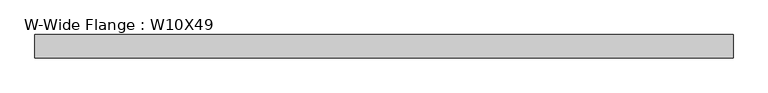
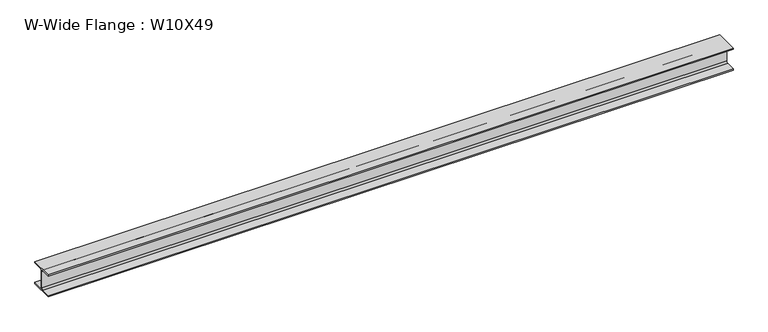
"""IFC4 building model written with IfcOpenShell, lengths in millimetres: beam geometry, W-Wide Flange : W10X49."""

from ifc_helpers import new_model, si_unit, point, frame, frame_2d, origin, place, context, project, spatial, polyline, circle_curve, trimmed, segment, composite_curve, outline, extrude, source, transform, mapped, element, save


def w_wide_flange_w10x49_ad4ce5ef(model_context):
    return source(origin(), model_context, "Body", "SweptSolid", [
        extrude(outline(composite_curve([segment(polyline([(127.0, -112.776), (127.0, -127.0), (-127.0, -127.0), (-127.0, -112.776), (-21.844, -112.776)]), True, "CONTINUOUS"), segment(trimmed(circle_curve(frame_2d((-21.844, -95.25)), 17.526), [point((-21.844, -112.776))], [point((-4.318, -95.25))], True, "CARTESIAN"), True, "CONTINUOUS"), segment(polyline([(-4.318, -95.25), (-4.318, 95.25)]), True, "CONTINUOUS"), segment(trimmed(circle_curve(frame_2d((-21.844, 95.25)), 17.526), [point((-4.318, 95.25))], [point((-21.844, 112.776))], True, "CARTESIAN"), True, "CONTINUOUS"), segment(polyline([(-21.844, 112.776), (-127.0, 112.776), (-127.0, 127.0), (127.0, 127.0), (127.0, 112.776), (21.844, 112.776)]), True, "CONTINUOUS"), segment(trimmed(circle_curve(frame_2d((21.844, 95.25)), 17.526), [point((21.844, 112.776))], [point((4.318, 95.25))], True, "CARTESIAN"), True, "CONTINUOUS"), segment(polyline([(4.318, 95.25), (4.318, -95.25)]), True, "CONTINUOUS"), segment(trimmed(circle_curve(frame_2d((21.844, -95.25)), 17.526), [point((4.318, -95.25))], [point((21.844, -112.776))], True, "CARTESIAN"), True, "CONTINUOUS"), segment(polyline([(21.844, -112.776), (127.0, -112.776)]), True, "CONTINUOUS")], self_intersect=False)), frame((-3764.7066406, 0.0, 0.0), z_axis=(1.0, 0.0, 0.0), x_axis=(0.0, 1.0, 0.0)), (0.0, 0.0, 1.0), 7529.4132813),
    ])


if __name__ == "__main__":
    model = new_model("IFC4")
    model_context = context("Model", 3, world=origin())
    ifc_project = project(units=[si_unit("LENGTHUNIT", "METRE", prefix="MILLI")], contexts=[model_context])
    site = spatial("IfcSite", under=ifc_project)
    building = spatial("IfcBuilding", under=site)
    placement = place(None, origin())
    w_wide_flange_w10x49_shape = w_wide_flange_w10x49_ad4ce5ef(model_context)
    element("IfcBeam", 1, ObjectType="W-Wide Flange : W10X49", at=placement, inside=building, context=model_context, shape_type="MappedRepresentation", body=[
        mapped(w_wide_flange_w10x49_shape, transform((0.0, 0.0, 0.0), x_axis=(1.0, 0.0, 0.0), y_axis=(0.0, 1.0, 0.0), z_axis=(0.0, 0.0, 1.0))),
    ])
    save(model, "model.ifc")

# Revit data of these elements
# Type "W-Wide Flange : W10X49"
#   Assembly Code = "B10"
#   W = 49
#   Length [instance default] = 1524 mm
#   bf = 254 mm
#   d = 254 mm
#   k = 31.75 mm
#   k2 = 17.526 mm
#   tf = 14.224 mm
#   tw = 8.636 mm
#   A = 0.0092903 m²
#   Structural Material [instance default] = Steel ASTM A992
# Element 1 (IfcBeam, "W-Wide Flange : W10X49")
#   Structural Material = Aluminum, Anodized Red
#   Materials on its faces: "Aluminum, Anodized Red"
# Materials
#   "Steel ASTM A992": class "Metal", colour RGB 128 0 0, transparency 0, Description = "Structural steel 50ksi", Cost = 0
#   "Aluminum, Anodized Red": class "Metal", colour RGB 120 120 120, transparency 0, Description = "Anodized aluminum, red", Cost = 0
